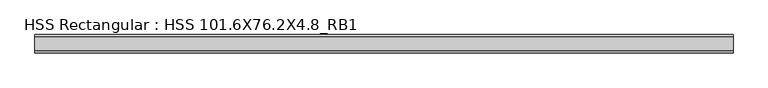
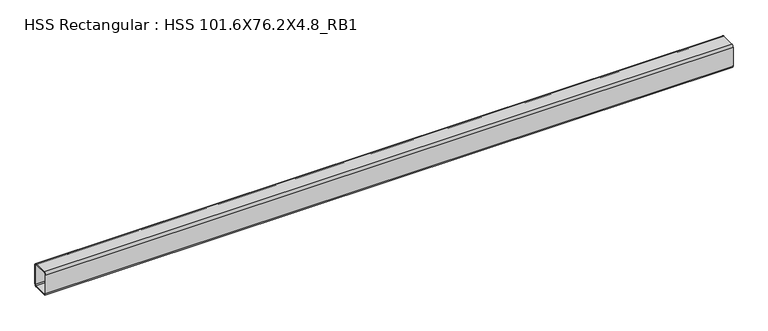
"""IFC4 building model written with IfcOpenShell, lengths in millimetres: beam geometry, HSS Rectangular : HSS 101.6X76.2X4.8_RB1."""

from ifc_helpers import new_model, si_unit, point, frame, frame_2d, origin, place, context, project, spatial, polyline, circle_curve, trimmed, segment, composite_curve, outline, extrude, source, transform, mapped, element, save


def hss_rectangular_hss_101_6x76_2x4_8_rb1_bb86ad5e(model_context):
    return source(origin(), model_context, "Body", "SweptSolid", [
        extrude(outline(composite_curve([segment(trimmed(circle_curve(frame_2d((-28.575, 41.275)), 9.525), [point((-38.1, 41.275))], [point((-28.575, 50.8))], False, "CARTESIAN"), True, "CONTINUOUS"), segment(polyline([(-28.575, 50.8), (28.575, 50.8)]), True, "CONTINUOUS"), segment(trimmed(circle_curve(frame_2d((28.575, 41.275)), 9.525), [point((28.575, 50.8))], [point((38.1, 41.275))], False, "CARTESIAN"), True, "CONTINUOUS"), segment(polyline([(38.1, 41.275), (38.1, -41.275)]), True, "CONTINUOUS"), segment(trimmed(circle_curve(frame_2d((28.575, -41.275)), 9.525), [point((38.1, -41.275))], [point((28.575, -50.8))], False, "CARTESIAN"), True, "CONTINUOUS"), segment(polyline([(28.575, -50.8), (-28.575, -50.8)]), True, "CONTINUOUS"), segment(trimmed(circle_curve(frame_2d((-28.575, -41.275)), 9.525), [point((-28.575, -50.8))], [point((-38.1, -41.275))], False, "CARTESIAN"), True, "CONTINUOUS"), segment(polyline([(-38.1, -41.275), (-38.1, 41.275)]), True, "CONTINUOUS")], self_intersect=False), holes=[composite_curve([segment(polyline([(28.575, 46.0375), (-28.575, 46.0375)]), True, "CONTINUOUS"), segment(trimmed(circle_curve(frame_2d((-28.575, 41.275)), 4.7625), [point((-28.575, 46.0375))], [point((-33.3375, 41.275))], True, "CARTESIAN"), True, "CONTINUOUS"), segment(polyline([(-33.3375, 41.275), (-33.3375, -41.275)]), True, "CONTINUOUS"), segment(trimmed(circle_curve(frame_2d((-28.575, -41.275)), 4.7625), [point((-33.3375, -41.275))], [point((-28.575, -46.0375))], True, "CARTESIAN"), True, "CONTINUOUS"), segment(polyline([(-28.575, -46.0375), (28.575, -46.0375)]), True, "CONTINUOUS"), segment(trimmed(circle_curve(frame_2d((28.575, -41.275)), 4.7625), [point((28.575, -46.0375))], [point((33.3375, -41.275))], True, "CARTESIAN"), True, "CONTINUOUS"), segment(polyline([(33.3375, -41.275), (33.3375, 41.275)]), True, "CONTINUOUS"), segment(trimmed(circle_curve(frame_2d((28.575, 41.275)), 4.7625), [point((33.3375, 41.275))], [point((28.575, 46.0375))], True, "CARTESIAN"), True, "CONTINUOUS")], self_intersect=False)]), frame((6083.0818722, 0.0, 0.0), z_axis=(1.0, 0.0, 0.0), x_axis=(0.0, 1.0, 0.0)), (0.0, 0.0, 1.0), 2885.3230622),
    ])


if __name__ == "__main__":
    model = new_model("IFC4")
    model_context = context("Model", 3, world=origin())
    ifc_project = project(units=[si_unit("LENGTHUNIT", "METRE", prefix="MILLI")], contexts=[model_context])
    site = spatial("IfcSite", under=ifc_project)
    building = spatial("IfcBuilding", under=site)
    placement = place(None, origin())
    hss_rectangular_hss_101_6x76_2x4_8_rb1_shape = hss_rectangular_hss_101_6x76_2x4_8_rb1_bb86ad5e(model_context)
    element("IfcBeam", 1, ObjectType="HSS Rectangular : HSS 101.6X76.2X4.8_RB1", at=placement, inside=building, context=model_context, shape_type="MappedRepresentation", body=[
        mapped(hss_rectangular_hss_101_6x76_2x4_8_rb1_shape, transform((0.0, 0.0, 0.0), x_axis=(1.0, 0.0, 0.0), y_axis=(0.0, 1.0, 0.0), z_axis=(0.0, 0.0, 1.0))),
    ])
    save(model, "model.ifc")

# Revit data of these elements
# Type "HSS Rectangular : HSS 101.6X76.2X4.8_RB1"
#   Section Name Key = "HSS 4X3X3/16"
#   Assembly Code = "B10"
#   Width = 7.62 cm
#   Wall Nominal Thickness = 0.4763 cm
#   Wall Design Thickness = 0.442 cm
#   Torsional Moment of Inertia = 260.561 cm⁴
#   Torsional Modulus = 61.2876 cm³
#   Section Area = 14.4516 cm²
#   Plastic Modulus weak axis = 40.3122 cm³
#   Plastic Modulus strong axis = 49.1612 cm³
#   Perimeter = 0.881482 m²/m
#   Outer Fillet = 0.9525 cm
#   Nominal Weight = 12.1285 kgf/m
#   Moment of Inertia weak axis = 131.529 cm⁴
#   Moment of Inertia strong axis = 205.202 cm⁴
#   Inner Fillet = 0.4763 cm
#   Height = 10.16 cm
#   Elastic Modulus weak axis = 34.4128 cm³
#   Elastic Modulus strong axis = 40.476 cm³
#   Centroid Vertical = 5.08 cm
#   Centroid Horizontal = 3.81 cm
#   Length [instance default] = 1524 mm
#   Structural Material [instance default] = Steel ASTM A500, Grade B, Rectangular and Square
#   Principal Axes Angle = 0
# Element 1 (IfcBeam, "HSS Rectangular : HSS 101.6X76.2X4.8_RB1")
#   Structural Material = Steel ASTM A992
#   Materials on its faces: "Steel ASTM A992"
# Materials
#   "Steel ASTM A500, Grade B, Rectangular and Square": class "Metal", colour RGB 199 199 199, transparency 0, Description = "Carbon steel", Cost = 0
#   "Steel ASTM A992": class "Metal", colour RGB 199 199 199, transparency 0, Description = "Structural steel 50ksi", Cost = 0
